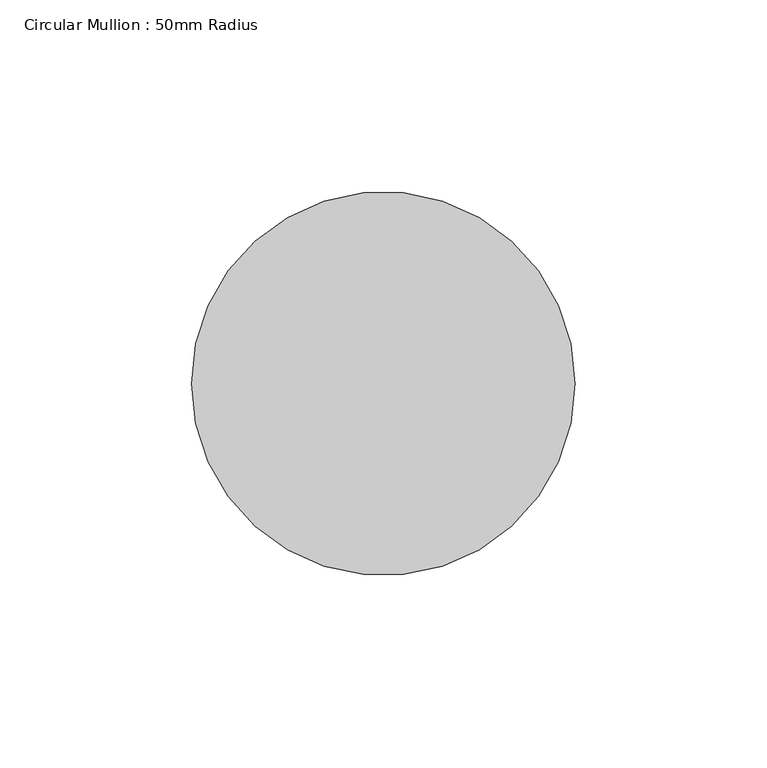
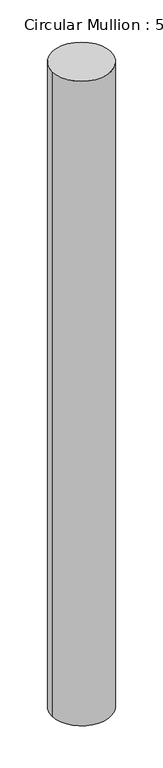
"""IFC4 building model written with IfcOpenShell, lengths in millimetres: member geometry, Circular Mullion : 50mm Radius."""

from ifc_helpers import new_model, si_unit, point, frame, origin, origin_2d, place, context, project, spatial, circle_curve, trimmed, segment, composite_curve, outline, extrude, source, transform, mapped, element, save


def circular_mullion_50mm_radius_ef2e3954(model_context):
    return source(origin(), model_context, "Body", "SweptSolid", [
        extrude(outline(composite_curve([segment(trimmed(circle_curve(origin_2d(), 50.0), [point((50.0, 0.0))], [point((-50.0, 0.0))], False, "CARTESIAN"), True, "CONTINUOUS"), segment(trimmed(circle_curve(origin_2d(), 50.0), [point((-50.0, 0.0))], [point((50.0, 0.0))], False, "CARTESIAN"), True, "CONTINUOUS")], self_intersect=False)), frame((0.0, 0.0, -1147.6468425), z_axis=(0.0, 0.0, 1.0), x_axis=(1.0, 0.0, 0.0)), (0.0, 0.0, 1.0), 1147.6468425),
    ])


if __name__ == "__main__":
    model = new_model("IFC4")
    model_context = context("Model", 3, world=origin())
    ifc_project = project(units=[si_unit("LENGTHUNIT", "METRE", prefix="MILLI")], contexts=[model_context])
    site = spatial("IfcSite", under=ifc_project)
    building = spatial("IfcBuilding", under=site)
    placement = place(None, origin())
    circular_mullion_50mm_radius_shape = circular_mullion_50mm_radius_ef2e3954(model_context)
    element("IfcMember", 1, ObjectType="Circular Mullion : 50mm Radius", at=placement, inside=building, context=model_context, shape_type="MappedRepresentation", body=[
        mapped(circular_mullion_50mm_radius_shape, transform((0.0, 0.0, 0.0), x_axis=(1.0, 0.0, 0.0), y_axis=(0.0, 1.0, 0.0), z_axis=(0.0, 0.0, 1.0))),
    ])
    save(model, "model.ifc")

# Revit data of these elements
# Type "Circular Mullion : 50mm Radius"
#   built-in parameter 1007350 = 0.164042 (stored number, unit not read)
# Element 1 (IfcMember, "Circular Mullion : 50mm Radius")
#   Materials on its faces: "Aluminium"
# Materials
#   "Aluminium": class "Metal", colour RGB 247 247 247, transparency 0, Description = "Aluminium 6061", Cost = 0
